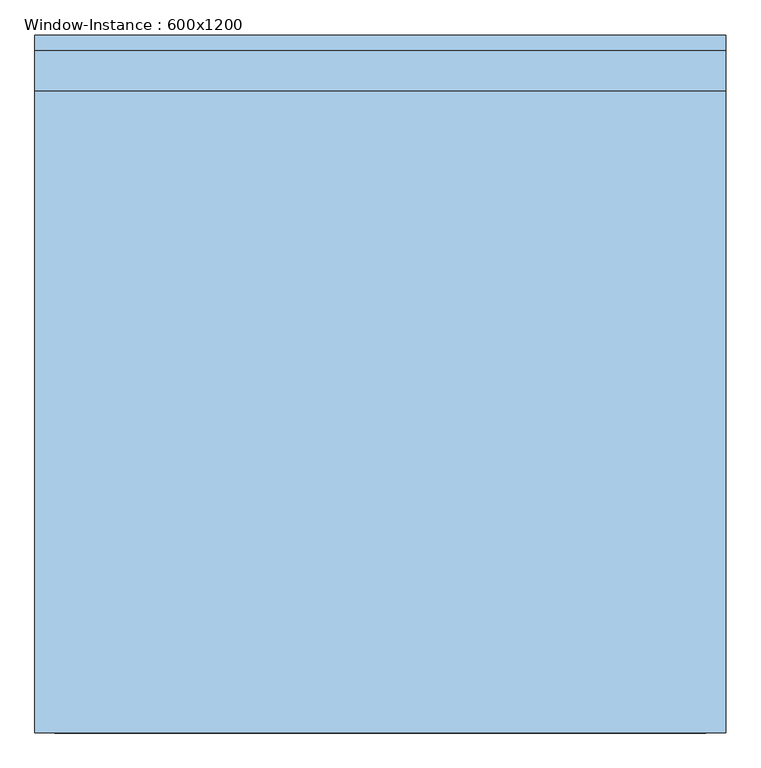
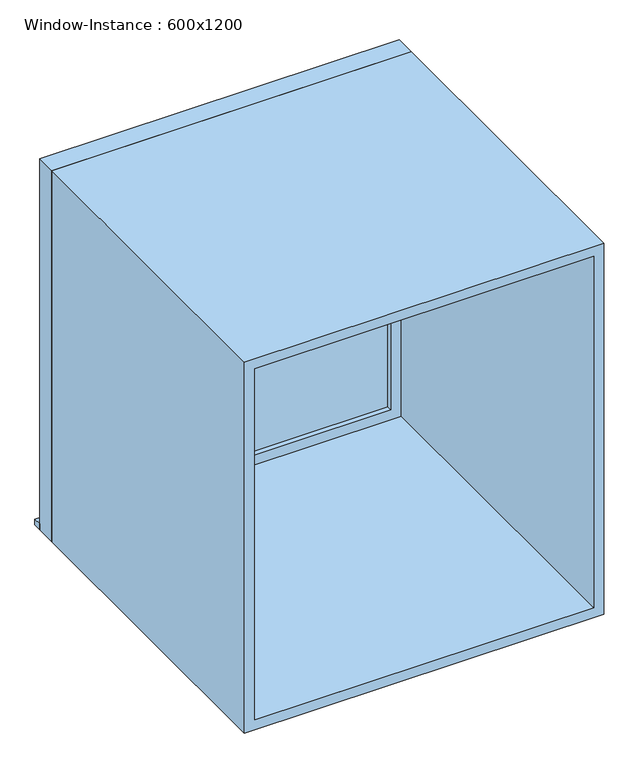
"""IFC4 building model written with IfcOpenShell, lengths in millimetres: window geometry, Window-Instance : 600x1200."""

from ifc_helpers import new_model, si_unit, frame, origin, place, context, project, spatial, polyline, outline, extrude, source, transform, mapped, element, save


def window_instance_600x1200_bc35079c(model_context):
    return source(origin(), model_context, "Body", "SweptSolid", [
        extrude(outline(polyline([(-588.1, 567.9), (511.9, 567.9), (511.9, 542.5), (-588.1, 542.5), (-588.1, 567.9)])), frame((0.0, 0.0, 900.0), z_axis=(0.0, 0.0, 1.0), x_axis=(1.0, 0.0, 0.0)), (0.0, 0.0, 1.0), 19.05),
        extrude(outline(polyline([(448.4, 493.925), (-524.6, 493.925), (-524.6, 506.625), (448.4, 506.625), (448.4, 493.925)])), frame((0.0, 0.0, 963.5), z_axis=(0.0, 0.0, 1.0), x_axis=(1.0, 0.0, 0.0)), (0.0, 0.0, 1.0), 1073.0),
        extrude(outline(polyline([(2080.95, -569.05), (919.05, -569.05), (919.05, 492.85), (2080.95, 492.85), (2080.95, -569.05)]), holes=[polyline([(2036.5, -524.6), (2036.5, 448.4), (963.5, 448.4), (963.5, -524.6), (2036.5, -524.6)])]), frame((0.0, 478.05, 0.0), z_axis=(0.0, 1.0, 0.0), x_axis=(0.0, 0.0, 1.0)), (0.0, 0.0, 1.0), 44.45),
        extrude(outline(polyline([(2100.0, -588.1), (900.0, -588.1), (900.0, 511.9), (2100.0, 511.9), (2100.0, -588.1)]), holes=[polyline([(2068.25, -556.35), (2068.25, 480.15), (931.75, 480.15), (931.75, -556.35), (2068.25, -556.35)])]), frame((0.0, -542.5, 0.0), z_axis=(0.0, 1.0, 0.0), x_axis=(0.0, 0.0, 1.0)), (0.0, 0.0, 1.0), 1020.55),
        extrude(outline(polyline([(2100.0, 511.9), (2100.0, -588.1), (900.0, -588.1), (900.0, 511.9), (2100.0, 511.9)]), holes=[polyline([(2080.95, 492.85), (919.05, 492.85), (919.05, -569.05), (2080.95, -569.05), (2080.95, 492.85)])]), frame((0.0, 478.05, 0.0), z_axis=(0.0, 1.0, 0.0), x_axis=(0.0, 0.0, 1.0)), (0.0, 0.0, 1.0), 64.45),
    ])


if __name__ == "__main__":
    model = new_model("IFC4")
    model_context = context("Model", 3, world=origin())
    ifc_project = project(units=[si_unit("LENGTHUNIT", "METRE", prefix="MILLI")], contexts=[model_context])
    site = spatial("IfcSite", under=ifc_project)
    building = spatial("IfcBuilding", under=site)
    placement = place(None, origin())
    window_instance_600x1200_shape = window_instance_600x1200_bc35079c(model_context)
    element("IfcWindow", 1, ObjectType="Window-Instance : 600x1200", at=placement, inside=building, context=model_context, shape_type="MappedRepresentation", body=[
        mapped(window_instance_600x1200_shape, transform((0.0, 0.0, 0.0), x_axis=(1.0, 0.0, 0.0), y_axis=(0.0, 1.0, 0.0), z_axis=(0.0, 0.0, 1.0))),
    ])
    save(model, "model.ifc")

# Revit data of these elements
# Type "Window-Instance : 600x1200"
#   Type Mark = "7"
#   Construction Type Id = "GSP4R"
#   Assembly Code = "B2020100"
#   Analytic Construction = "1/8 in Pilkington single glazing"
#   Visual Light Transmittance = 0.9
#   Thermal Resistance (R) = 0.149095 (m²·K)/W
#   Solar Heat Gain Coefficient = 0.86
#   Heat Transfer Coefficient (U) = 6.70716 W/(m²·K)
#   Height [instance default] = 1200 mm
#   Default Sill Height = 900 mm
#   Width [instance default] = 600 mm
#   Window Inset = 20 mm
#   Glass Pane Material = WW-EC-GL-Storefront
#   Sash Material = WW-EC-RGB-White
#   Wall Closure = (empty or 0)
# Element 1 (IfcWindow, "Window-Instance : 600x1200")
#   Width = 1100 mm
#   Materials on its faces: "WW-EC-RGB-White", "WW-EC-GL-Storefront"
# Materials
#   "WW-EC-GL-Storefront": class "Glass", colour RGB 236 240 239, transparency 0.85, Description = "Storefront Glass", Cost = 0
#   "WW-EC-RGB-White": class "Generic", colour RGB 255 255 255, transparency 0, Comments = "If region requests off-white, swith asset color to RGB 231-228-220", Description = "Generic Color", Cost = 0
